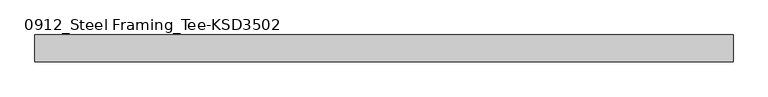
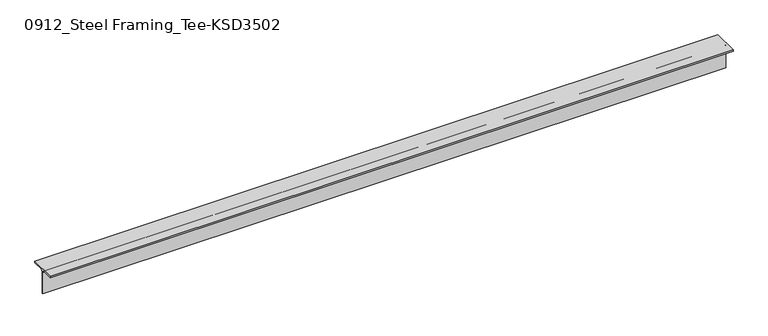
"""IFC4 building model written with IfcOpenShell, lengths in millimetres: member geometry, 0912_Steel Framing_Tee-KSD3502 : H_SB_ASB_CT-150x150x6.5x9."""

from ifc_helpers import new_model, si_unit, point, frame, frame_2d, origin, place, context, project, spatial, polyline, circle_curve, trimmed, segment, composite_curve, outline, extrude, source, transform, mapped, element, save


def member_0912_steel_framing_tee_ksd3502_03d888ff(model_context):
    return source(origin(), model_context, "Body", "SweptSolid", [
        extrude(outline(composite_curve([segment(polyline([(75.0, 75.0), (75.0, 66.0), (16.25, 66.0)]), True, "CONTINUOUS"), segment(trimmed(circle_curve(frame_2d((16.25, 53.0)), 13.0), [point((16.25, 66.0))], [point((3.25, 53.0))], True, "CARTESIAN"), True, "CONTINUOUS"), segment(polyline([(3.25, 53.0), (3.25, -75.0), (-3.25, -75.0), (-3.25, 53.0)]), True, "CONTINUOUS"), segment(trimmed(circle_curve(frame_2d((-16.25, 53.0)), 13.0), [point((-3.25, 53.0))], [point((-16.25, 66.0))], True, "CARTESIAN"), True, "CONTINUOUS"), segment(polyline([(-16.25, 66.0), (-75.0, 66.0), (-75.0, 75.0), (75.0, 75.0)]), True, "CONTINUOUS")], self_intersect=False)), frame((-1965.45, 0.0, 0.0), z_axis=(1.0, 0.0, 0.0), x_axis=(0.0, 1.0, 0.0)), (0.0, 0.0, 1.0), 3898.3),
    ])


if __name__ == "__main__":
    model = new_model("IFC4")
    model_context = context("Model", 3, world=origin())
    ifc_project = project(units=[si_unit("LENGTHUNIT", "METRE", prefix="MILLI")], contexts=[model_context])
    site = spatial("IfcSite", under=ifc_project)
    building = spatial("IfcBuilding", under=site)
    placement = place(None, origin())
    member_0912_steel_framing_tee_ksd3502_shape = member_0912_steel_framing_tee_ksd3502_03d888ff(model_context)
    element("IfcMember", 1, ObjectType="0912_Steel Framing_Tee-KSD3502 : H_SB_ASB_CT-150x150x6.5x9", at=placement, inside=building, context=model_context, shape_type="MappedRepresentation", body=[
        mapped(member_0912_steel_framing_tee_ksd3502_shape, transform((0.0, 0.0, 0.0), x_axis=(1.0, 0.0, 0.0), y_axis=(0.0, 1.0, 0.0), z_axis=(0.0, 0.0, 1.0))),
    ])
    save(model, "model.ifc")

# Revit data of these elements
# Type "0912_Steel Framing_Tee-KSD3502 : H_SB_ASB_CT-150x150x6.5x9"
#   H_WM Code_1 = "S01AA003-00001 | Main Steel Structure Fabrication Work | Shelter/Building | Light Steel - Standard (30KG/M>Weight) | Material: (   )"
#   H_WM Code_2 = "S03AA029-00001 | Main Steel Structure Erection Work | Shelter/Building | Light Steel (30KG/M>Weight) | Material: (   )"
#   H_WM Code_3 = "S01AA010-00001 | Main Steel Structure Fabrication Work | Shelter/Building | Steel Painting/Coating | for Non-Fireproofed Steel Surface, Surface Preparation, Primer, Second & Final Coat | Material: (   )"
#   H_Q'ty Cal Type Tag = "SB-Q2"
#   Width = 15.0 cm
#   Web Thickness = 0.65 cm
#   Web Fillet = 1.3 cm
#   Section Area = 23.39 cm²
#   Perimeter = 0.60 m²/m
#   Nominal Weight = 18.40 kgf/m
#   Height = 15.0 cm
#   Flange Thickness = 0.9 cm
#   Centroid Vertical = 7.5 cm
#   Centroid Horizontal = 7.5 cm
#   Length [instance default] = 1.5000 m
#   Structural Material [instance default] = Steel, 45-345
#   Warping Constant = (empty or 0)
#   Torsional Moment of Inertia = 0
#   Section Name Key = ""
#   Plastic Modulus weak axis = 0
#   Plastic Modulus strong axis = 0
#   Moment of Inertia weak axis = 0
#   Moment of Inertia strong axis = 0
#   Elastic Modulus weak axis = 0
#   Elastic Modulus strong axis = 0
#   Bolt Spacing = 0
#   Assembly Code = ""
# Element 1 (IfcMember, "0912_Steel Framing_Tee-KSD3502 : H_SB_ASB_CT-150x150x6.5x9")
#   Structural Material = none
# Materials
#   "Steel, 45-345": class "Metal", colour RGB 189 187 185, transparency 0, Description = "Steel 345 MPa", Cost = 0
